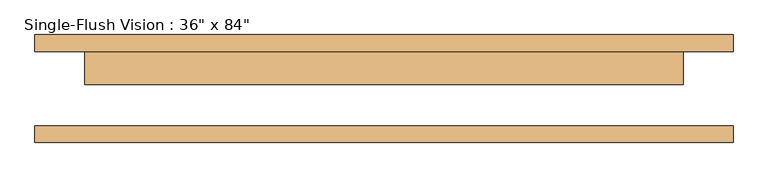
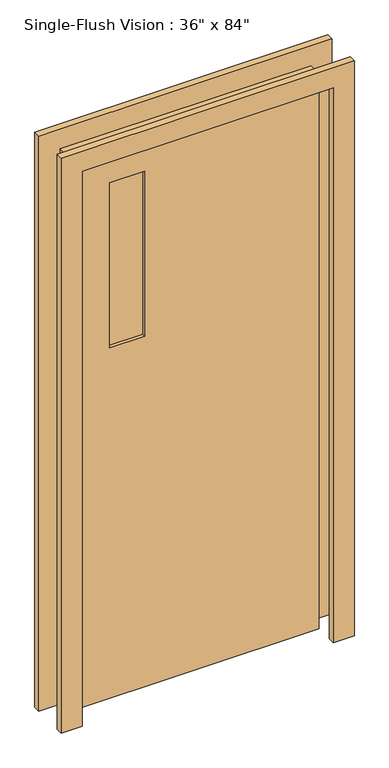
"""IFC4 building model written with IfcOpenShell, lengths in millimetres: door geometry."""

from ifc_helpers import new_model, si_unit, frame, origin, place, context, project, spatial, polyline, outline, extrude, source, transform, mapped, element, save


def door_fde454a0(model_context):
    return source(origin(), model_context, "Body", "SweptSolid", [
        extrude(outline(polyline([(2209.8, -533.4), (0.0, -533.4), (0.0, -457.2), (2133.6, -457.2), (2133.6, 457.2), (0.0, 457.2), (0.0, 533.4), (2209.8, 533.4), (2209.8, -533.4)])), frame((0.0, 57.15, 0.0), z_axis=(0.0, 1.0, 0.0), x_axis=(0.0, 0.0, 1.0)), (0.0, 0.0, 1.0), 25.4),
        extrude(outline(polyline([(2133.6, 457.2), (0.0, 457.2), (0.0, 533.4), (2209.8, 533.4), (2209.8, -533.4), (0.0, -533.4), (0.0, -457.2), (2133.6, -457.2), (2133.6, 457.2)])), frame((0.0, -82.55, 0.0), z_axis=(0.0, 1.0, 0.0), x_axis=(0.0, 0.0, 1.0)), (0.0, 0.0, 1.0), 25.4),
        extrude(outline(polyline([(-177.8, 19.05), (-304.8, 19.05), (-304.8, 25.4), (-177.8, 25.4), (-177.8, 19.05)])), frame((0.0, 0.0, 1346.2), z_axis=(0.0, 0.0, 1.0), x_axis=(1.0, 0.0, 0.0)), (0.0, 0.0, 1.0), 635.0),
        extrude(outline(polyline([(-177.8, 38.1), (-304.8, 38.1), (-304.8, 44.45), (-177.8, 44.45), (-177.8, 38.1)])), frame((0.0, 0.0, 1346.2), z_axis=(0.0, 0.0, 1.0), x_axis=(1.0, 0.0, 0.0)), (0.0, 0.0, 1.0), 635.0),
        extrude(outline(polyline([(2133.6, -457.2), (0.0, -457.2), (0.0, 457.2), (2133.6, 457.2), (2133.6, -457.2)]), holes=[polyline([(1981.2, -304.8), (1981.2, -177.8), (1346.2, -177.8), (1346.2, -304.8), (1981.2, -304.8)])]), frame((0.0, 6.35, 0.0), z_axis=(0.0, 1.0, 0.0), x_axis=(0.0, 0.0, 1.0)), (0.0, 0.0, 1.0), 50.8),
    ])


if __name__ == "__main__":
    model = new_model("IFC4")
    model_context = context("Model", 3, world=origin())
    ifc_project = project(units=[si_unit("LENGTHUNIT", "METRE", prefix="MILLI")], contexts=[model_context])
    site = spatial("IfcSite", under=ifc_project)
    building = spatial("IfcBuilding", under=site)
    placement = place(None, origin())
    door_shape = door_fde454a0(model_context)
    element("IfcDoor", 1, ObjectType="Single-Flush Vision : 36\" x 84\"", at=placement, inside=building, context=model_context, shape_type="MappedRepresentation", body=[
        mapped(door_shape, transform((0.0, 0.0, 0.0), x_axis=(1.0, 0.0, 0.0), y_axis=(0.0, 1.0, 0.0), z_axis=(0.0, 0.0, 1.0))),
    ])
    save(model, "model.ifc")

# Revit data of these elements
# Type "Single-Flush Vision : 36\" x 84\""
#   Type Mark = "21"
#   Assembly Code = "C1020"
#   Thickness = 0' - 2"
#   Height = 7' - 0"
#   Lite Height = 2' - 1"
#   Lite Width = 0' - 5"
#   Side Rail = 0' - 6"
#   Top Rail = 0' - 6"
#   Trim Projection = 0' - 1"
#   Trim Width Ext. = 0' - 3"
#   Trim Width Int. = 0' - 3"
#   Width = 3' - 0"
#   Function = 0
#   Door Material = Door - Panel
#   Frame Material = Door - Frame
#   Wall Closure = (empty or 0)
# Element 1 (IfcDoor, "Single-Flush Vision : 36\" x 84\"")
#   Materials on its faces: "Door - Frame", "Glass", "Door - Panel"
# Materials
#   "Door - Panel": class "Wood", colour RGB 230 193 158, transparency 0, Cost = 0
#   "Door - Frame": class "Paint", colour RGB 113 0 0, transparency 0, Cost = 0
#   "Glass": class "Glass", colour RGB 0 128 192, transparency 0.75, Cost = 0
